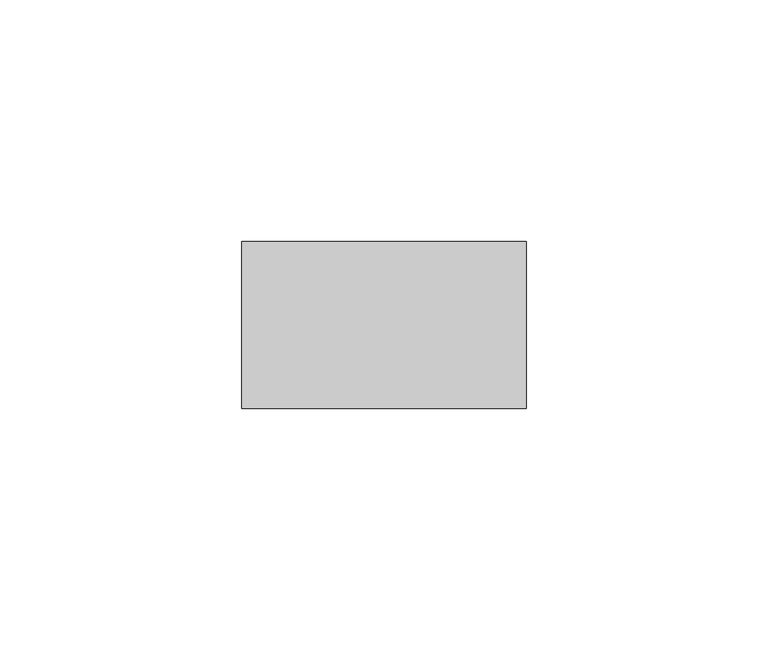
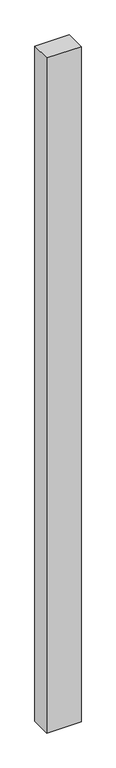
"""IFC4 building model written with IfcOpenShell, lengths in millimetres: proxy geometry, Inner panel:Inner panel:1:Inner panel:1 : Inner panel:Inner panel:300324:300043:Inner panel:1:Inner panel:1 : Inner panel:Inner panel:300324:300043 : Inner panel:Inner panel:1:Inner panel:1 : Inner panel:Inner panel:300324:300043:43 : Inner panel:Inner panel:1:Inner panel:1 : Inner panel:Inner panel:300324:300043:Inner panel:1:Inner panel:1 : Inner panel:Inner panel:300324:300043 : Inner panel:Inner panel:1:Inner panel:1 : Inner panel:Inner panel:300324:300043:300031."""

from ifc_helpers import new_model, si_unit, frame, origin, place, context, project, spatial, polyline, outline, extrude, source, transform, mapped, element, save


def generic_models_d2030a4c(model_context):
    return source(origin(), model_context, "Body", "SweptSolid", [
        extrude(outline(polyline([(667266.1522107, -568237.7769044), (667325.0617239, -568237.7769044), (667325.0617239, -568272.3525973), (667266.1522107, -568272.3525973), (667266.1522107, -568237.7769044)])), frame((0.0, 0.0, 4946.65), z_axis=(0.0, 0.0, 1.0), x_axis=(1.0, 0.0, 0.0)), (0.0, 0.0, 1.0), 1219.2),
    ])


if __name__ == "__main__":
    model = new_model("IFC4")
    model_context = context("Model", 3, world=origin())
    ifc_project = project(units=[si_unit("LENGTHUNIT", "METRE", prefix="MILLI")], contexts=[model_context])
    site = spatial("IfcSite", under=ifc_project)
    building = spatial("IfcBuilding", under=site)
    placement = place(None, origin())
    generic_models_shape = generic_models_d2030a4c(model_context)
    element("IfcBuildingElementProxy", 1, Name="Inner panel:Inner panel:1:Inner panel:1 : Inner panel:Inner panel:300324:300043:Inner panel:1:Inner panel:1 : Inner panel:Inner panel:300324:300043 : Inner panel:Inner panel:1:Inner panel:1 : Inner panel:Inner panel:300324:300043:43 : Inner panel:Inner panel:1:Inner panel:1 : Inner panel:Inner panel:300324:300043:Inner panel:1:Inner panel:1 : Inner panel:Inner panel:300324:300043 : Inner panel:Inner panel:1:Inner panel:1 : Inner panel:Inner panel:300324:300043:300031", ObjectType="Inner panel:Inner panel:1:Inner panel:1 : Inner panel:Inner panel:300324:300043:Inner panel:1:Inner panel:1 : Inner panel:Inner panel:300324:300043 : Inner panel:Inner panel:1:Inner panel:1 : Inner panel:Inner panel:300324:300043:43 : Inner panel:Inner panel:1:Inner panel:1 : Inner panel:Inner panel:300324:300043:Inner panel:1:Inner panel:1 : Inner panel:Inner panel:300324:300043 : Inner panel:Inner panel:1:Inner panel:1 : Inner panel:Inner panel:300324:300043:300031", at=placement, inside=building, context=model_context, shape_type="MappedRepresentation", body=[
        mapped(generic_models_shape, transform((0.0, 0.0, 0.0), x_axis=(1.0, 0.0, 0.0), y_axis=(0.0, 1.0, 0.0), z_axis=(0.0, 0.0, 1.0))),
    ])
    save(model, "model.ifc")

# Revit data of these elements
# Type "Inner panel:Inner panel:1:Inner panel:1 : Inner panel:Inner panel:300324:300043:Inner panel:1:Inner panel:1 : Inner panel:Inner panel:300324:300043 : Inner panel:Inner panel:1:Inner panel:1 : Inner panel:Inner panel:300324:300043:43 : Inner panel:Inner panel:1:Inner panel:1 : Inner panel:Inner panel:300324:300043:Inner panel:1:Inner panel:1 : Inner panel:Inner panel:300324:300043 : Inner panel:Inner panel:1:Inner panel:1 : Inner panel:Inner panel:300324:300043:300031"
#   NameOverride = "Inner panel:Inner panel:1:Inner panel:1 : Inner panel:Inner panel:300324:300043:Inner panel:1:Inner panel:1 : Inner panel:Inner panel:300324:300043 : Inner panel:Inner panel:1:Inner panel:1 : Inner panel:Inner panel:300324:300043:300031"
#   ObjectTypeOverride = "Inner panel:1:Inner panel:1 : Inner panel:Inner panel:300324:300043 : Inner panel:Inner panel:1:Inner panel:1 : Inner panel:Inner panel:300324:300043"
#   Reference = "Inner panel"
#   Tag = "300031"
# Element 1 (IfcBuildingElementProxy, "Inner panel:Inner panel:1:Inner panel:1 : Inner panel:Inner panel:300324:300043:Inner panel:1:Inner panel:1 : Inner panel:Inner panel:300324:300043 : Inner panel:Inner panel:1:Inner panel:1 : Inner panel:Inner panel:300324:300043:43 : Inner panel:Inner panel:1:Inner panel:1 : Inner panel:Inner panel:300324:300043:Inner panel:1:Inner panel:1 : Inner panel:Inner panel:300324:300043 : Inner panel:Inner panel:1:Inner panel:1 : Inner panel:Inner panel:300324:300043:300031")
#   Materials on its faces: "FIRE RETARDTANT WOOD BLOCKING - SIZE AS NECESSARY"
# Materials
#   "FIRE RETARDTANT WOOD BLOCKING - SIZE AS NECESSARY": class "Wood", colour RGB 144 113 62, transparency 0, Description = "Pinus Echinata", Cost = 0
